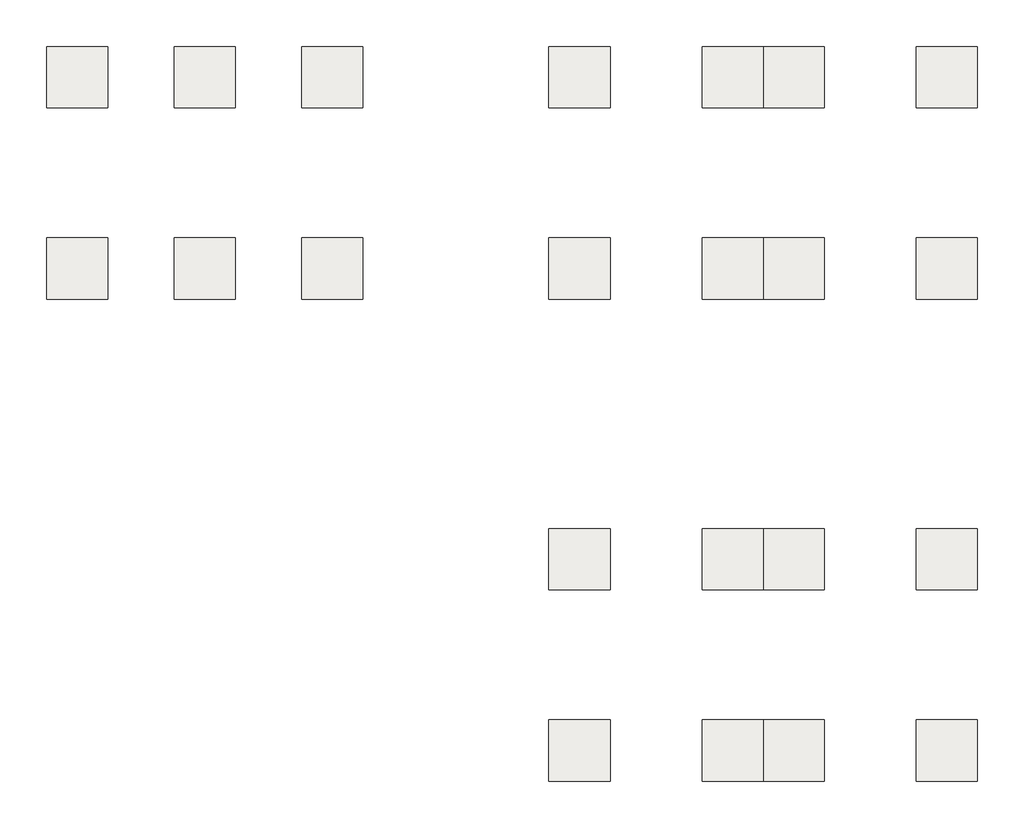
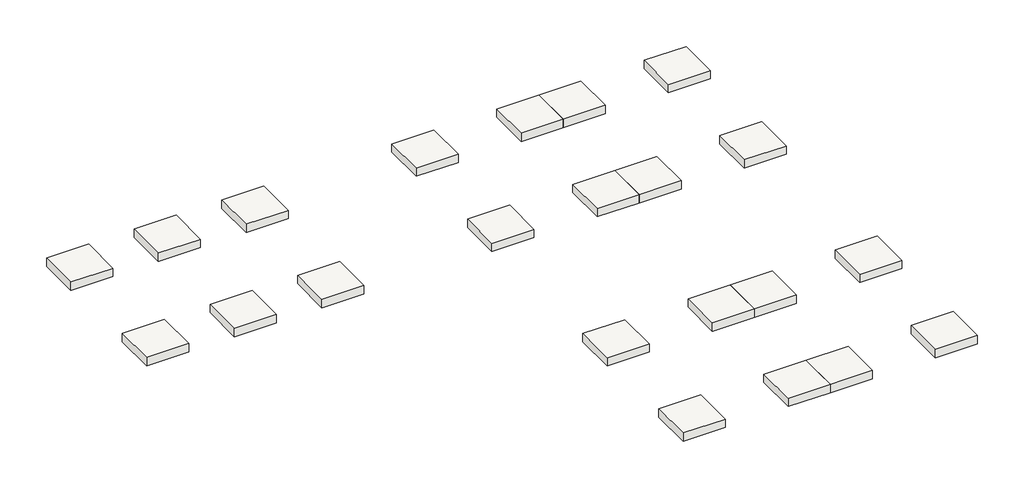
# One storey: 22 slabs.
"""IFC4 building model written with IfcOpenShell, lengths in millimetres."""

import ifcopenshell
import ifcopenshell.guid

model = None  # the IFC model being written
_history = None  # IfcOwnerHistory: only IFC2X3 demands one
_inside = {}  # id of a spatial element -> (the spatial element, [elements in it])
_under = {}  # id of a project, library or spatial element -> (it, [spatial elements below it])
_declared = {}  # id of a project -> (the project, [libraries it declares])
_typed = {}  # id of a type object -> (the type object, [elements of that type])
_made_of = {}  # id of a material, layer set ... -> (it, [elements and type objects made of it])


def new_model(schema):
    """Start an empty IFC model of exactly this schema.

    Asked for "IFC4X3", IfcOpenShell would pick the latest addendum, in which some entities
    have other attributes; the version numbers below select the first issue.
    IFC2X3 requires an IfcOwnerHistory on every rooted entity: one is made here for all.
    """
    global model, _history
    if schema == "IFC4X3":
        model = ifcopenshell.file(schema_version=(4, 3, 0, 0))
    else:
        model = ifcopenshell.file(schema=schema)
    _inside.clear()
    _under.clear()
    _declared.clear()
    _typed.clear()
    _made_of.clear()
    _history = None
    if model.schema == "IFC2X3":
        org = make("IfcOrganization", Name="unknown")
        user = make(
            "IfcPersonAndOrganization",
            ThePerson=make("IfcPerson", FamilyName="unknown"),
            TheOrganization=org,
        )
        app = make(
            "IfcApplication",
            ApplicationDeveloper=org,
            Version="unknown",
            ApplicationFullName="unknown",
            ApplicationIdentifier="unknown",
        )
        _history = make(
            "IfcOwnerHistory",
            OwningUser=user,
            OwningApplication=app,
            ChangeAction="ADDED",
            CreationDate=0,
        )
    return model


def make(cls, **values):
    """One entity of the class cls with the attributes given. An attribute that is None is left unset."""
    return model.create_entity(
        cls, **{name: value for name, value in values.items() if value is not None}
    )


def rooted(cls, **values):
    """An entity with a GlobalId (a new one), such as an element, a storey or a relation."""
    return make(cls, GlobalId=ifcopenshell.guid.new(), OwnerHistory=_history, **values)


def si_unit(unit_type, name, prefix=None):
    """IfcSIUnit, for example si_unit("LENGTHUNIT", "METRE", prefix="MILLI")."""
    return make("IfcSIUnit", UnitType=unit_type, Prefix=prefix, Name=name)


def assignment(units):
    """IfcUnitAssignment: the units of a project."""
    return None if units is None else make("IfcUnitAssignment", Units=units)


def point(xyz):
    """IfcCartesianPoint."""
    return None if xyz is None else make("IfcCartesianPoint", Coordinates=xyz)


def direction(xyz):
    """IfcDirection."""
    return None if xyz is None else make("IfcDirection", DirectionRatios=xyz)


def frame(location, z_axis=None, x_axis=None):
    """IfcAxis2Placement3D, a coordinate frame: its origin and axes. An axis left out is left unset."""
    return make(
        "IfcAxis2Placement3D",
        Location=point(location),
        Axis=direction(z_axis),
        RefDirection=direction(x_axis),
    )


def origin():
    """The frame at (0, 0, 0) with its axes left unset."""
    return frame((0.0, 0.0, 0.0))


def place(relative_to, where):
    """IfcLocalPlacement: puts the frame where relative to a parent placement (None: the world)."""
    return make(
        "IfcLocalPlacement", PlacementRelTo=relative_to, RelativePlacement=where
    )


def context(
    kind, dimensions, precision=None, world=None, true_north=None, identifier=None
):
    """IfcGeometricRepresentationContext, for example the 3D "Model" context."""
    return make(
        "IfcGeometricRepresentationContext",
        ContextIdentifier=identifier,
        ContextType=kind,
        CoordinateSpaceDimension=dimensions,
        Precision=precision,
        WorldCoordinateSystem=world,
        TrueNorth=true_north,
    )


def project(units=None, contexts=None):
    """IfcProject with its units and contexts."""
    return rooted(
        "IfcProject",
        Name="project",
        RepresentationContexts=contexts,
        UnitsInContext=assignment(units),
    )


def spatial(cls, under=None, at=None, **own):
    """A site, building, storey or space (cls), placed at a placement, below another one or the project."""
    s = rooted(cls, ObjectPlacement=at, **own)
    if under is not None:
        _under.setdefault(under.id(), (under, []))[1].append(s)
    return s


def polyline(points):
    """IfcPolyline through the points."""
    return make("IfcPolyline", Points=[point(p) for p in points])


def outline(outer, holes=None, kind="AREA"):
    """IfcArbitraryClosedProfileDef: a profile drawn as a closed curve; with holes, ...WithVoids."""
    if holes is None:
        return make("IfcArbitraryClosedProfileDef", ProfileType=kind, OuterCurve=outer)
    return make(
        "IfcArbitraryProfileDefWithVoids",
        ProfileType=kind,
        OuterCurve=outer,
        InnerCurves=holes,
    )


def extrude(swept, where, along, depth):
    """IfcExtrudedAreaSolid: the profile swept, set in the frame where, extruded along a direction by depth."""
    return make(
        "IfcExtrudedAreaSolid",
        SweptArea=swept,
        Position=where,
        ExtrudedDirection=direction(along),
        Depth=depth,
    )


def shape(context_of_items, identifier, shape_type, items):
    """IfcShapeRepresentation: the items that make up one representation, for example the "Body"."""
    return make(
        "IfcShapeRepresentation",
        ContextOfItems=context_of_items,
        RepresentationIdentifier=identifier,
        RepresentationType=shape_type,
        Items=items,
    )


def source(mapping_origin, context_of_items, identifier, shape_type, items):
    """IfcRepresentationMap: a shape defined once, which mapped items show again and again."""
    return make(
        "IfcRepresentationMap",
        MappingOrigin=mapping_origin,
        MappedRepresentation=shape(context_of_items, identifier, shape_type, items),
    )


def transform(
    local_origin,
    x_axis=None,
    y_axis=None,
    z_axis=None,
    scale=None,
    scale2=None,
    scale3=None,
    uniform=True,
):
    """IfcCartesianTransformationOperator3D, or its non-uniform kind. x_axis, y_axis, z_axis: its Axis1, 2, 3."""
    if uniform:
        return make(
            "IfcCartesianTransformationOperator3D",
            Axis1=direction(x_axis),
            Axis2=direction(y_axis),
            LocalOrigin=point(local_origin),
            Scale=scale,
            Axis3=direction(z_axis),
        )
    return make(
        "IfcCartesianTransformationOperator3DnonUniform",
        Axis1=direction(x_axis),
        Axis2=direction(y_axis),
        LocalOrigin=point(local_origin),
        Scale=scale,
        Axis3=direction(z_axis),
        Scale2=scale2,
        Scale3=scale3,
    )


def mapped(mapping_source, mapping_target):
    """IfcMappedItem: shows the shape of a source again, moved by a transform."""
    return make(
        "IfcMappedItem", MappingSource=mapping_source, MappingTarget=mapping_target
    )


def made_of(thing, what):
    """Note that an element or type object is made of a material, layer set ...; save() writes the relation."""
    if what is not None:
        _made_of.setdefault(what.id(), (what, []))[1].append(thing)
    return thing


def element(
    cls,
    number,
    at=None,
    inside=None,
    cuts=None,
    type_object=None,
    material=None,
    context=None,
    identifier="Body",
    shape_type=None,
    held_by="IfcProductDefinitionShape",
    body=None,
    shapes=None,
    **own,
):
    """One element of the class cls, such as IfcWall. Its Tag is "e" and its number.

    at: its placement. inside: the storey or other place that contains it. cuts: it is an
    opening in that element (IfcRelVoidsElement). A single representation is given by context,
    identifier, shape_type and body (its items); several are given by shapes. held_by: the class
    of the entity that holds the representations. save() writes the other relations.
    """
    e = rooted(cls, Tag="e%d" % number, ObjectPlacement=at, **own)
    if body is not None:
        shapes = [shape(context, identifier, shape_type, body)]
    if shapes is not None:
        e.Representation = make(held_by, Representations=shapes)
    if inside is not None:
        _inside.setdefault(inside.id(), (inside, []))[1].append(e)
    if cuts is not None:
        rooted(
            "IfcRelVoidsElement", RelatingBuildingElement=cuts, RelatedOpeningElement=e
        )
    if type_object is not None:
        _typed.setdefault(type_object.id(), (type_object, []))[1].append(e)
    return made_of(e, material)


def aggregate(whole, parts):
    """IfcRelAggregates: a whole, such as a stair, and the parts it consists of."""
    return rooted("IfcRelAggregates", RelatingObject=whole, RelatedObjects=parts)


def save(model, path):
    """Write the relations noted so far, then the file.

    IfcRelAggregates (storeys below a building ...), IfcRelContainedInSpatialStructure (elements
    in a storey), IfcRelDefinesByType, IfcRelAssociatesMaterial and IfcRelDeclares: one each for
    every whole, place, type object, material and project.
    """
    for whole, parts in _under.values():
        aggregate(whole, parts)
    for where, things in _inside.values():
        rooted(
            "IfcRelContainedInSpatialStructure",
            RelatedElements=things,
            RelatingStructure=where,
        )
    for kind, things in _typed.values():
        rooted("IfcRelDefinesByType", RelatedObjects=things, RelatingType=kind)
    for what, things in _made_of.values():
        rooted("IfcRelAssociatesMaterial", RelatedObjects=things, RelatingMaterial=what)
    for by, libraries in _declared.values():
        rooted("IfcRelDeclares", RelatingContext=by, RelatedDefinitions=libraries)
    model.write(path)


def ft112_footing_rectangular_ft112_2400x2400x500_5fe39465(model_context):
    return source(origin(), model_context, "Body", "SweptSolid", [
        extrude(outline(polyline([(1200.0, 1200.0), (1200.0, -1200.0), (-1200.0, -1200.0), (-1200.0, 1200.0), (1200.0, 1200.0)])), frame((0.0, 0.0, -500.0), z_axis=(0.0, 0.0, 1.0), x_axis=(1.0, 0.0, 0.0)), (0.0, 0.0, 1.0), 500.0),
    ])


model = new_model("IFC4")

# Units and contexts
model_context = context("Model", 3, world=origin())
ifc_project = project(units=[si_unit("LENGTHUNIT", "METRE", prefix="MILLI")], contexts=[model_context])

# Site, building, storey
site = spatial("IfcSite", under=ifc_project)
building = spatial("IfcBuilding", under=site)
storey = spatial("IfcBuildingStorey", under=building, Name="B.O.F", Elevation=-1800.0)

# Slabs
placement = place(None, origin())
element("IfcSlab", 1, ObjectType="FT112-Footing-Rectangular : FT112_2400x2400x500", at=placement, inside=storey, context=model_context, shape_type="SweptSolid", body=[
    extrude(outline(polyline([(26820.0, 14699.5208589), (26820.0, 12299.5208589), (24420.0, 12299.5208589), (24420.0, 14699.5208589), (26820.0, 14699.5208589)])), frame((0.0, 0.0, -1800.0), z_axis=(0.0, 0.0, 1.0), x_axis=(1.0, 0.0, 0.0)), (0.0, 0.0, 1.0), 500.0),
])
element("IfcSlab", 2, ObjectType="FT112-Footing-Rectangular : FT112_2400x2400x500", at=placement, inside=storey, context=model_context, shape_type="SweptSolid", body=[
    extrude(outline(polyline([(26820.0, 22199.5208589), (26820.0, 19799.5208589), (24420.0, 19799.5208589), (24420.0, 22199.5208589), (26820.0, 22199.5208589)])), frame((0.0, 0.0, -1800.0), z_axis=(0.0, 0.0, 1.0), x_axis=(1.0, 0.0, 0.0)), (0.0, 0.0, 1.0), 500.0),
])
element("IfcSlab", 3, ObjectType="FT112-Footing-Rectangular : FT112_2400x2400x500", at=placement, inside=storey, context=model_context, shape_type="SweptSolid", body=[
    extrude(outline(polyline([(29220.0, 14699.5208589), (29220.0, 12299.5208589), (26820.0, 12299.5208589), (26820.0, 14699.5208589), (29220.0, 14699.5208589)])), frame((0.0, 0.0, -1800.0), z_axis=(0.0, 0.0, 1.0), x_axis=(1.0, 0.0, 0.0)), (0.0, 0.0, 1.0), 500.0),
])
element("IfcSlab", 4, ObjectType="FT112-Footing-Rectangular : FT112_2400x2400x500", at=placement, inside=storey, context=model_context, shape_type="SweptSolid", body=[
    extrude(outline(polyline([(29220.0, 22199.5208589), (29220.0, 19799.5208589), (26820.0, 19799.5208589), (26820.0, 22199.5208589), (29220.0, 22199.5208589)])), frame((0.0, 0.0, -1800.0), z_axis=(0.0, 0.0, 1.0), x_axis=(1.0, 0.0, 0.0)), (0.0, 0.0, 1.0), 500.0),
])
element("IfcSlab", 5, ObjectType="FT112-Footing-Rectangular : FT112_2400x2400x500", at=placement, inside=storey, context=model_context, shape_type="SweptSolid", body=[
    extrude(outline(polyline([(35220.0, 14699.5208589), (35220.0, 12299.5208589), (32820.0, 12299.5208589), (32820.0, 14699.5208589), (35220.0, 14699.5208589)])), frame((0.0, 0.0, -1800.0), z_axis=(0.0, 0.0, 1.0), x_axis=(1.0, 0.0, 0.0)), (0.0, 0.0, 1.0), 500.0),
])
element("IfcSlab", 6, ObjectType="FT112-Footing-Rectangular : FT112_2400x2400x500", at=placement, inside=storey, context=model_context, shape_type="SweptSolid", body=[
    extrude(outline(polyline([(35220.0, 22199.5208589), (35220.0, 19799.5208589), (32820.0, 19799.5208589), (32820.0, 22199.5208589), (35220.0, 22199.5208589)])), frame((0.0, 0.0, -1800.0), z_axis=(0.0, 0.0, 1.0), x_axis=(1.0, 0.0, 0.0)), (0.0, 0.0, 1.0), 500.0),
])
element("IfcSlab", 7, ObjectType="FT112-Footing-Rectangular : FT112_2400x2400x500", at=placement, inside=storey, context=model_context, shape_type="SweptSolid", body=[
    extrude(outline(polyline([(18420.0, 14699.5208589), (20820.0, 14699.5208589), (20820.0, 12299.5208589), (18420.0, 12299.5208589), (18420.0, 14699.5208589)])), frame((0.0, 0.0, -1800.0), z_axis=(0.0, 0.0, 1.0), x_axis=(1.0, 0.0, 0.0)), (0.0, 0.0, 1.0), 500.0),
])
element("IfcSlab", 8, ObjectType="FT112-Footing-Rectangular : FT112_2400x2400x500", at=placement, inside=storey, context=model_context, shape_type="SweptSolid", body=[
    extrude(outline(polyline([(18420.0, 22199.5208589), (20820.0, 22199.5208589), (20820.0, 19799.5208589), (18420.0, 19799.5208589), (18420.0, 22199.5208589)])), frame((0.0, 0.0, -1800.0), z_axis=(0.0, 0.0, 1.0), x_axis=(1.0, 0.0, 0.0)), (0.0, 0.0, 1.0), 500.0),
])
element("IfcSlab", 9, ObjectType="FT112-Footing-Rectangular : FT112_2400x2400x500", at=placement, inside=storey, context=model_context, shape_type="SweptSolid", body=[
    extrude(outline(polyline([(26820.0, -4200.4791411), (26820.0, -6600.4791411), (24420.0, -6600.4791411), (24420.0, -4200.4791411), (26820.0, -4200.4791411)])), frame((0.0, 0.0, -1800.0), z_axis=(0.0, 0.0, 1.0), x_axis=(1.0, 0.0, 0.0)), (0.0, 0.0, 1.0), 500.0),
])
element("IfcSlab", 10, ObjectType="FT112-Footing-Rectangular : FT112_2400x2400x500", at=placement, inside=storey, context=model_context, shape_type="SweptSolid", body=[
    extrude(outline(polyline([(26820.0, 3299.5208589), (26820.0, 899.5208589), (24420.0, 899.5208589), (24420.0, 3299.5208589), (26820.0, 3299.5208589)])), frame((0.0, 0.0, -1800.0), z_axis=(0.0, 0.0, 1.0), x_axis=(1.0, 0.0, 0.0)), (0.0, 0.0, 1.0), 500.0),
])
element("IfcSlab", 11, ObjectType="FT112-Footing-Rectangular : FT112_2400x2400x500", at=placement, inside=storey, context=model_context, shape_type="SweptSolid", body=[
    extrude(outline(polyline([(29220.0, -4200.4791411), (29220.0, -6600.4791411), (26820.0, -6600.4791411), (26820.0, -4200.4791411), (29220.0, -4200.4791411)])), frame((0.0, 0.0, -1800.0), z_axis=(0.0, 0.0, 1.0), x_axis=(1.0, 0.0, 0.0)), (0.0, 0.0, 1.0), 500.0),
])
element("IfcSlab", 12, ObjectType="FT112-Footing-Rectangular : FT112_2400x2400x500", at=placement, inside=storey, context=model_context, shape_type="SweptSolid", body=[
    extrude(outline(polyline([(29220.0, 3299.5208589), (29220.0, 899.5208589), (26820.0, 899.5208589), (26820.0, 3299.5208589), (29220.0, 3299.5208589)])), frame((0.0, 0.0, -1800.0), z_axis=(0.0, 0.0, 1.0), x_axis=(1.0, 0.0, 0.0)), (0.0, 0.0, 1.0), 500.0),
])
element("IfcSlab", 13, ObjectType="FT112-Footing-Rectangular : FT112_2400x2400x500", at=placement, inside=storey, context=model_context, shape_type="SweptSolid", body=[
    extrude(outline(polyline([(35220.0, -4200.4791411), (35220.0, -6600.4791411), (32820.0, -6600.4791411), (32820.0, -4200.4791411), (35220.0, -4200.4791411)])), frame((0.0, 0.0, -1800.0), z_axis=(0.0, 0.0, 1.0), x_axis=(1.0, 0.0, 0.0)), (0.0, 0.0, 1.0), 500.0),
])
element("IfcSlab", 14, ObjectType="FT112-Footing-Rectangular : FT112_2400x2400x500", at=placement, inside=storey, context=model_context, shape_type="SweptSolid", body=[
    extrude(outline(polyline([(35220.0, 3299.5208589), (35220.0, 899.5208589), (32820.0, 899.5208589), (32820.0, 3299.5208589), (35220.0, 3299.5208589)])), frame((0.0, 0.0, -1800.0), z_axis=(0.0, 0.0, 1.0), x_axis=(1.0, 0.0, 0.0)), (0.0, 0.0, 1.0), 500.0),
])
element("IfcSlab", 15, ObjectType="FT112-Footing-Rectangular : FT112_2400x2400x500", at=placement, inside=storey, context=model_context, shape_type="SweptSolid", body=[
    extrude(outline(polyline([(18420.0, -4200.4791411), (20820.0, -4200.4791411), (20820.0, -6600.4791411), (18420.0, -6600.4791411), (18420.0, -4200.4791411)])), frame((0.0, 0.0, -1800.0), z_axis=(0.0, 0.0, 1.0), x_axis=(1.0, 0.0, 0.0)), (0.0, 0.0, 1.0), 500.0),
])
element("IfcSlab", 16, ObjectType="FT112-Footing-Rectangular : FT112_2400x2400x500", at=placement, inside=storey, context=model_context, shape_type="SweptSolid", body=[
    extrude(outline(polyline([(18420.0, 3299.5208589), (20820.0, 3299.5208589), (20820.0, 899.5208589), (18420.0, 899.5208589), (18420.0, 3299.5208589)])), frame((0.0, 0.0, -1800.0), z_axis=(0.0, 0.0, 1.0), x_axis=(1.0, 0.0, 0.0)), (0.0, 0.0, 1.0), 500.0),
])
ft112_footing_rectangular_ft112_2400x2400x500_shape = ft112_footing_rectangular_ft112_2400x2400x500_5fe39465(model_context)
element("IfcSlab", 17, ObjectType="FT112-Footing-Rectangular : FT112_2400x2400x500", at=placement, inside=storey, context=model_context, shape_type="MappedRepresentation", body=[
    mapped(ft112_footing_rectangular_ft112_2400x2400x500_shape, transform((4920.0, 13499.5208589, -1300.0), x_axis=(1.0, 0.0, 0.0), y_axis=(0.0, 1.0, 0.0), z_axis=(0.0, 0.0, 1.0))),
])
element("IfcSlab", 18, ObjectType="FT112-Footing-Rectangular : FT112_2400x2400x500", at=placement, inside=storey, context=model_context, shape_type="MappedRepresentation", body=[
    mapped(ft112_footing_rectangular_ft112_2400x2400x500_shape, transform((9920.0, 13499.5208589, -1300.0), x_axis=(1.0, 0.0, 0.0), y_axis=(0.0, 1.0, 0.0), z_axis=(0.0, 0.0, 1.0))),
])
element("IfcSlab", 19, ObjectType="FT112-Footing-Rectangular : FT112_2400x2400x500", at=placement, inside=storey, context=model_context, shape_type="MappedRepresentation", body=[
    mapped(ft112_footing_rectangular_ft112_2400x2400x500_shape, transform((9920.0, 20999.5208589, -1300.0), x_axis=(1.0, 0.0, 0.0), y_axis=(0.0, 1.0, 0.0), z_axis=(0.0, 0.0, 1.0))),
])
element("IfcSlab", 20, ObjectType="FT112-Footing-Rectangular : FT112_2400x2400x500", at=placement, inside=storey, context=model_context, shape_type="MappedRepresentation", body=[
    mapped(ft112_footing_rectangular_ft112_2400x2400x500_shape, transform((4920.0, 20999.5208589, -1300.0), x_axis=(1.0, 0.0, 0.0), y_axis=(0.0, 1.0, 0.0), z_axis=(0.0, 0.0, 1.0))),
])
element("IfcSlab", 21, ObjectType="FT112-Footing-Rectangular : FT112_2400x2400x500", at=placement, inside=storey, context=model_context, shape_type="MappedRepresentation", body=[
    mapped(ft112_footing_rectangular_ft112_2400x2400x500_shape, transform((-80.0, 20999.5208589, -1300.0), x_axis=(1.0, 0.0, 0.0), y_axis=(0.0, 1.0, 0.0), z_axis=(0.0, 0.0, 1.0))),
])
element("IfcSlab", 22, ObjectType="FT112-Footing-Rectangular : FT112_2400x2400x500", at=placement, inside=storey, context=model_context, shape_type="MappedRepresentation", body=[
    mapped(ft112_footing_rectangular_ft112_2400x2400x500_shape, transform((-80.0, 13499.5208589, -1300.0), x_axis=(1.0, 0.0, 0.0), y_axis=(0.0, 1.0, 0.0), z_axis=(0.0, 0.0, 1.0))),
])

save(model, "model.ifc")

# Revit data of these elements
# Project information
#   Building Name = "Main Gate Security"
#   Project Status = "Project Status"
#   Client Name = "현대엔지니어링"
#   Project Address = "서울시 종로구 율곡로 75(계동)"
#   Project Name = "Therma Visayas Energy Project"
#   Project Number = "001"
# Grids (mm)
#   "B": line (5000, 25626.165) -> (5000, 10142.075)
#   "C": line (10000, 25626.165) -> (10000, 10142.075)
#   "A": line (0, 25626.165) -> (0, 10142.075)
#   "5": line (3500, 10142.075) -> (3500, 25626.165)
#   "6": line (7500, 10142.075) -> (7500, 25626.165)
#   "10": line (14956.387, 18199.521) -> (-5363.617, 18199.521)
#   "1": line (-5363.617, 13499.521) -> (13263.593, 13499.521)
#   "2": line (-5363.617, 20999.521) -> (13263.593, 20999.521)
# Type "FT112-Footing-Rectangular : FT112_2400x2400x500"
#   Description = "UG Shallow Foundation"
#   Width = 2400 mm
#   Length = 2400 mm
#   Foundation Thickness = 500 mm
#   hec_material3 [instance default] = none
#   hec_material2 [instance default] = A03AE056-00001_Bitumen/Bituminous/Asphalt Coating
#   hec_material1 [instance default] = A03AC035-00001_Form Work (3 times in use)_Flat
#   Structural Material [instance default] = A03AC032-00007_Structural Concrete_Type1_25MPa-30Mpa
#   Assembly Code = ""
# Elements 1, 2, 3, 4, 5, 6, 7, 8, 9, 10, 11, 12, 13, 14, 15, 16, 17, 18, 19, 20 (IfcSlab, "FT112-Footing-Rectangular : FT112_2400x2400x500")
#   Comments = ""
#   F01) Building Name = "Main Gate House"
#   F11) Project Building Tag_Type-1 = "Common"
#   F12) Project Building Tag_Type-2 = "Common"
#   F13) Project Facility Code = "Facility Code"
#   F21) Structural Type = "Concrete"
#   F31) Standard Building Code = "IBC"
#   F41) Discipline = "AR"
#   F51) Plan Start Date-Engineering = "2015-01-01"
#   F52) Plan Finish Date-Engineering = "2015-12-31"
#   F53) Duration = "365"
#   F54) Actual Start Date-Engineering = "2015-01-01"
#   F55) Actual Finish Date-Engineering = "2015-12-31"
#   F61) Plan Start Date-Construction = "2016-08-19"
#   F62) Plan Finish Date-Construction = "2017-01-31"
#   F64) Actual Start Date-Construction = "2016-08-19"
#   F63) Duration = "202"
#   F65) Actual Finish Date-Construction = "2017-01-31"
#   F91) Plant Type = "CFPP"
#   F92) KKS Structures, Building = "UYF"
#   P01) Project Name = "TVEP"
#   P02) Project Configuration = "CFB Boiler x 2(Foster Wheeler) + STG x 2(Alstom, 150MW)"
#   P03) Project Abbreviation = "TVEP"
#   P04) Project Code = "BEPH1402"
#   P05) Project Stage = "In operation"
#   P06) Project Location = "Sito Looc, Barangay Bato, Toledo City in Philippines"
#   P07) Project Owner = "Therma Visayas, Inc."
#   P08) Project O.E = "Flour"
#   P09) Project Schedule = "ITB Issueing Date : 2013.07.30\r\nSite Survey : 2013.08.19-20\r\nBid Closing Date : 2013.11.29\r\nPreferred Bidder Notice 접수 : 2014.04.27\r\nTarget award date : 2014 05\r\nLOA 접수 : 2014.05.21\r\nSigning Ceremony : 2014.05.30"
#   P10) Basic Wind Speed = "55.6 m/s"
#   P11) Seismic = "NSCP 2010, Zone 4 (PGA : 0.4g)"
#   P12) Soil = "Sc"
#   P13) Soil Capacity = "100kN/m2"
#   P14) Pile Capacity = "PHC(D400) : 1200kN"
#   W00) Work Master Code = "A03AC032-00007"
#   W01) Work Master_Lv1 = "Concrete Work"
#   W02) Work Master_Lv2 = "Substructure Work"
#   W03) Work Master_Spec.1 = "Cement Type-1"
#   W04) Work Master_Spec.2 = "25MPa < F'c (Cylinder Strength) ≤ 30MPa"
#   W11) Activity ID = "C02AGB010"
#   W12) Activity Name = "Main Gate Security Building - Building Foundation"
#   W13) Plan Start Date = "2016-08-19"
#   W14) Plan Finish Date = "2016-09-22"
#   W15) Duration = "26"
#   W16) Actual Start Date = "2016-08-19"
#   W17) Actual Finish Date = "2016-09-22"
#   R02) Unit Price = 0
#   Structural Material = A03AC032-00007_Structural Concrete_Type1_25MPa-30Mpa
#   hec_material3 = none
#   hec_material2 = none
#   hec_material1 = none
#   Phase Created = New Construction
#   Materials on its faces: "A03AC032-00007_Structural Concrete_Type1_25MPa-30Mpa"
# Elements 21, 22 (IfcSlab, "FT112-Footing-Rectangular : FT112_2400x2400x500")
#   Comments = ""
#   F01) Building Name = "Main Gate House"
#   F11) Project Building Tag_Type-1 = "Common"
#   F12) Project Building Tag_Type-2 = "Common"
#   F13) Project Facility Code = "Facility Code"
#   F21) Structural Type = "Concrete"
#   F31) Standard Building Code = "IBC"
#   F41) Discipline = "AR"
#   F51) Plan Start Date-Engineering = "2015-01-01"
#   F52) Plan Finish Date-Engineering = "2015-12-31"
#   F53) Duration = "365"
#   F54) Actual Start Date-Engineering = "2015-01-01"
#   F55) Actual Finish Date-Engineering = "2015-12-31"
#   F61) Plan Start Date-Construction = "2016-08-19"
#   F62) Plan Finish Date-Construction = "2017-01-31"
#   F64) Actual Start Date-Construction = "2016-08-19"
#   F63) Duration = "202"
#   F65) Actual Finish Date-Construction = "2017-01-31"
#   F91) Plant Type = "CFPP"
#   F92) KKS Structures, Building = "UYF"
#   P01) Project Name = "TVEP"
#   P02) Project Configuration = "CFB Boiler x 2(Foster Wheeler) + STG x 2(Alstom, 150MW)"
#   P03) Project Abbreviation = "TVEP"
#   P04) Project Code = "BEPH1402"
#   P05) Project Stage = "In operation"
#   P06) Project Location = "Sito Looc, Barangay Bato, Toledo City in Philippines"
#   P07) Project Owner = "Therma Visayas, Inc."
#   P08) Project O.E = "Flour"
#   P09) Project Schedule = "ITB Issueing Date : 2013.07.30\r\nSite Survey : 2013.08.19-20\r\nBid Closing Date : 2013.11.29\r\nPreferred Bidder Notice 접수 : 2014.04.27\r\nTarget award date : 2014 05\r\nLOA 접수 : 2014.05.21\r\nSigning Ceremony : 2014.05.30"
#   P10) Basic Wind Speed = "55.6 m/s"
#   P11) Seismic = "NSCP 2010, Zone 4 (PGA : 0.4g)"
#   P12) Soil = "Sc"
#   P13) Soil Capacity = "100kN/m2"
#   P14) Pile Capacity = "PHC(D400) : 1200kN"
#   W00) Work Master Code = "A03AC032-00007"
#   W01) Work Master_Lv1 = "Concrete Work"
#   W02) Work Master_Lv2 = "Substructure Work"
#   W03) Work Master_Spec.1 = "Cement Type-1"
#   W04) Work Master_Spec.2 = "25MPa < F'c (Cylinder Strength) ≤ 30MPa"
#   W11) Activity ID = "C02AGB010"
#   W12) Activity Name = "Main Gate Security Building - Building Foundation"
#   W13) Plan Start Date = "2016-08-19"
#   W14) Plan Finish Date = "2016-09-22"
#   W15) Duration = "26"
#   W16) Actual Start Date = "2016-08-19"
#   W17) Actual Finish Date = "2016-09-22"
#   R02) Unit Price = 0
#   Structural Material = A03AC032-00007_Structural Concrete_Type1_25MPa-30Mpa
#   hec_material3 = none
#   hec_material2 = none
#   hec_material1 = A03AD035-2505_Form Work_3 times
#   Phase Created = New Construction
#   Materials on its faces: "A03AC032-00007_Structural Concrete_Type1_25MPa-30Mpa"
# Materials
#   "A03AE056-00001_Bitumen/Bituminous/Asphalt Coating": class "Generic", colour RGB 17 17 17, transparency 0, Description = "Damp-proofing", W00) Work Master Code = "A03AE056-00001", W01) Work Master_Lv1 = "Concrete Work", W02) Work Master_Lv2 = "Concrete Protective Coating (U/G)", W03) Work Master_Spec.1 = "Bitumen/Bituminous/Asphalt Coating", Cost = 0
#   "A03AC035-00001_Form Work (3 times in use)_Flat": class "Wood", colour RGB 149 120 74, transparency 0, Description = "Plywood", W00) Work Master Code = "A03AC035-00001", W01) Work Master_Lv1 = "Concrete Work", W02) Work Master_Lv2 = "Substructure Work", W03) Work Master_Spec.1 = "Form Work (3 times in use)", W04) Work Master_Spec.2 = "Flat Form", W05) Work Master_Spec.3 = "Dressed Lumber, Plywood or Steel Form(Wood Planks are not Allowed) incl. Chamfer", Cost = 0
#   "A03AC032-00007_Structural Concrete_Type1_25MPa-30Mpa": class "Concrete", colour RGB 176 176 176, transparency 0, Keynote = "09910.A1", Description = "Reinf. Conc.", W00) Work Master Code = "A03AC032-00007", W01) Work Master_Lv1 = "Concrete Work", W02) Work Master_Lv2 = "Substructure Work", W03) Work Master_Spec.1 = "Structural Concrete", W04) Work Master_Spec.2 = "Cement Type-1", W05) Work Master_Spec.3 = "25MPa < F'c (Cylinder Strength) ≤ 30MPa", Cost = 0
#   "A03AD035-2505_Form Work_3 times": class "Wood", colour RGB 149 120 74, transparency 0, Description = "Plywood", W00) Work Master Code = "A03AD035-2505", W01) Work Master_Lv1 = "Concrete Work", W02) Work Master_Lv2 = "Superstructure Work", W03) Work Master_Spec.1 = "Form Work (3 times in use)", W04) Work Master_Spec.2 = "Flat Form", W05) Work Master_Spec.3 = "Dressed Lumber, Plywood or Steel Form(Wood Planks are not Allowed) incl. Chamfer", Cost = 0
